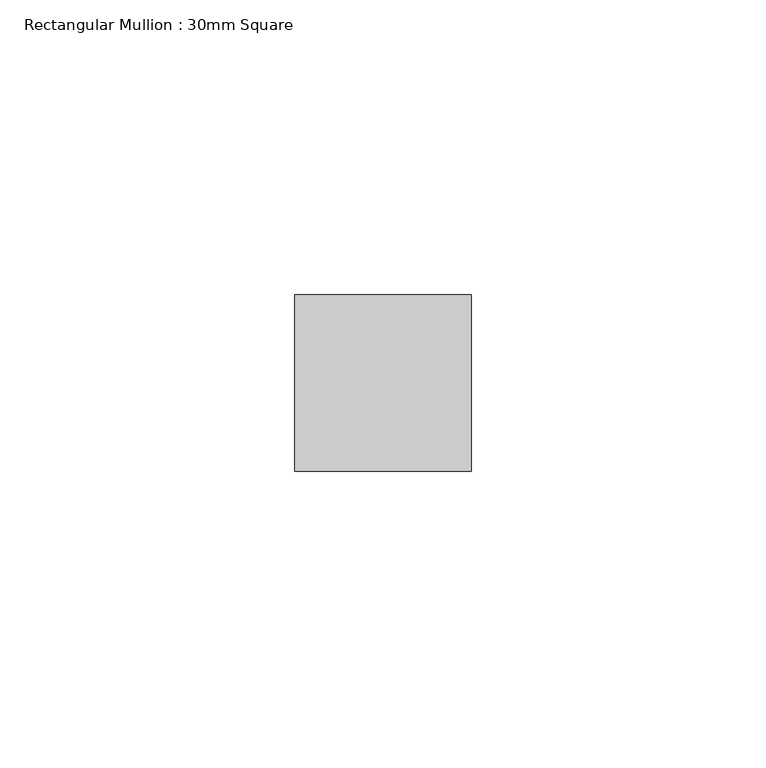
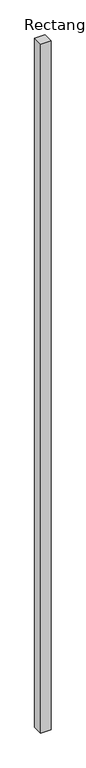
"""IFC4 building model written with IfcOpenShell, lengths in millimetres: member geometry, Rectangular Mullion : 30mm Square."""

import ifcopenshell
import ifcopenshell.guid

model = None  # the IFC model being written
_history = None  # IfcOwnerHistory: only IFC2X3 demands one
_inside = {}  # id of a spatial element -> (the spatial element, [elements in it])
_under = {}  # id of a project, library or spatial element -> (it, [spatial elements below it])
_declared = {}  # id of a project -> (the project, [libraries it declares])
_typed = {}  # id of a type object -> (the type object, [elements of that type])
_made_of = {}  # id of a material, layer set ... -> (it, [elements and type objects made of it])


def new_model(schema):
    """Start an empty IFC model of exactly this schema.

    Asked for "IFC4X3", IfcOpenShell would pick the latest addendum, in which some entities
    have other attributes; the version numbers below select the first issue.
    IFC2X3 requires an IfcOwnerHistory on every rooted entity: one is made here for all.
    """
    global model, _history
    if schema == "IFC4X3":
        model = ifcopenshell.file(schema_version=(4, 3, 0, 0))
    else:
        model = ifcopenshell.file(schema=schema)
    _inside.clear()
    _under.clear()
    _declared.clear()
    _typed.clear()
    _made_of.clear()
    _history = None
    if model.schema == "IFC2X3":
        org = make("IfcOrganization", Name="unknown")
        user = make(
            "IfcPersonAndOrganization",
            ThePerson=make("IfcPerson", FamilyName="unknown"),
            TheOrganization=org,
        )
        app = make(
            "IfcApplication",
            ApplicationDeveloper=org,
            Version="unknown",
            ApplicationFullName="unknown",
            ApplicationIdentifier="unknown",
        )
        _history = make(
            "IfcOwnerHistory",
            OwningUser=user,
            OwningApplication=app,
            ChangeAction="ADDED",
            CreationDate=0,
        )
    return model


def make(cls, **values):
    """One entity of the class cls with the attributes given. An attribute that is None is left unset."""
    return model.create_entity(
        cls, **{name: value for name, value in values.items() if value is not None}
    )


def rooted(cls, **values):
    """An entity with a GlobalId (a new one), such as an element, a storey or a relation."""
    return make(cls, GlobalId=ifcopenshell.guid.new(), OwnerHistory=_history, **values)


def si_unit(unit_type, name, prefix=None):
    """IfcSIUnit, for example si_unit("LENGTHUNIT", "METRE", prefix="MILLI")."""
    return make("IfcSIUnit", UnitType=unit_type, Prefix=prefix, Name=name)


def assignment(units):
    """IfcUnitAssignment: the units of a project."""
    return None if units is None else make("IfcUnitAssignment", Units=units)


def point(xyz):
    """IfcCartesianPoint."""
    return None if xyz is None else make("IfcCartesianPoint", Coordinates=xyz)


def direction(xyz):
    """IfcDirection."""
    return None if xyz is None else make("IfcDirection", DirectionRatios=xyz)


def frame(location, z_axis=None, x_axis=None):
    """IfcAxis2Placement3D, a coordinate frame: its origin and axes. An axis left out is left unset."""
    return make(
        "IfcAxis2Placement3D",
        Location=point(location),
        Axis=direction(z_axis),
        RefDirection=direction(x_axis),
    )


def origin():
    """The frame at (0, 0, 0) with its axes left unset."""
    return frame((0.0, 0.0, 0.0))


def place(relative_to, where):
    """IfcLocalPlacement: puts the frame where relative to a parent placement (None: the world)."""
    return make(
        "IfcLocalPlacement", PlacementRelTo=relative_to, RelativePlacement=where
    )


def context(
    kind, dimensions, precision=None, world=None, true_north=None, identifier=None
):
    """IfcGeometricRepresentationContext, for example the 3D "Model" context."""
    return make(
        "IfcGeometricRepresentationContext",
        ContextIdentifier=identifier,
        ContextType=kind,
        CoordinateSpaceDimension=dimensions,
        Precision=precision,
        WorldCoordinateSystem=world,
        TrueNorth=true_north,
    )


def project(units=None, contexts=None):
    """IfcProject with its units and contexts."""
    return rooted(
        "IfcProject",
        Name="project",
        RepresentationContexts=contexts,
        UnitsInContext=assignment(units),
    )


def spatial(cls, under=None, at=None, **own):
    """A site, building, storey or space (cls), placed at a placement, below another one or the project."""
    s = rooted(cls, ObjectPlacement=at, **own)
    if under is not None:
        _under.setdefault(under.id(), (under, []))[1].append(s)
    return s


def polyline(points):
    """IfcPolyline through the points."""
    return make("IfcPolyline", Points=[point(p) for p in points])


def outline(outer, holes=None, kind="AREA"):
    """IfcArbitraryClosedProfileDef: a profile drawn as a closed curve; with holes, ...WithVoids."""
    if holes is None:
        return make("IfcArbitraryClosedProfileDef", ProfileType=kind, OuterCurve=outer)
    return make(
        "IfcArbitraryProfileDefWithVoids",
        ProfileType=kind,
        OuterCurve=outer,
        InnerCurves=holes,
    )


def extrude(swept, where, along, depth):
    """IfcExtrudedAreaSolid: the profile swept, set in the frame where, extruded along a direction by depth."""
    return make(
        "IfcExtrudedAreaSolid",
        SweptArea=swept,
        Position=where,
        ExtrudedDirection=direction(along),
        Depth=depth,
    )


def shape(context_of_items, identifier, shape_type, items):
    """IfcShapeRepresentation: the items that make up one representation, for example the "Body"."""
    return make(
        "IfcShapeRepresentation",
        ContextOfItems=context_of_items,
        RepresentationIdentifier=identifier,
        RepresentationType=shape_type,
        Items=items,
    )


def source(mapping_origin, context_of_items, identifier, shape_type, items):
    """IfcRepresentationMap: a shape defined once, which mapped items show again and again."""
    return make(
        "IfcRepresentationMap",
        MappingOrigin=mapping_origin,
        MappedRepresentation=shape(context_of_items, identifier, shape_type, items),
    )


def transform(
    local_origin,
    x_axis=None,
    y_axis=None,
    z_axis=None,
    scale=None,
    scale2=None,
    scale3=None,
    uniform=True,
):
    """IfcCartesianTransformationOperator3D, or its non-uniform kind. x_axis, y_axis, z_axis: its Axis1, 2, 3."""
    if uniform:
        return make(
            "IfcCartesianTransformationOperator3D",
            Axis1=direction(x_axis),
            Axis2=direction(y_axis),
            LocalOrigin=point(local_origin),
            Scale=scale,
            Axis3=direction(z_axis),
        )
    return make(
        "IfcCartesianTransformationOperator3DnonUniform",
        Axis1=direction(x_axis),
        Axis2=direction(y_axis),
        LocalOrigin=point(local_origin),
        Scale=scale,
        Axis3=direction(z_axis),
        Scale2=scale2,
        Scale3=scale3,
    )


def mapped(mapping_source, mapping_target):
    """IfcMappedItem: shows the shape of a source again, moved by a transform."""
    return make(
        "IfcMappedItem", MappingSource=mapping_source, MappingTarget=mapping_target
    )


def made_of(thing, what):
    """Note that an element or type object is made of a material, layer set ...; save() writes the relation."""
    if what is not None:
        _made_of.setdefault(what.id(), (what, []))[1].append(thing)
    return thing


def element(
    cls,
    number,
    at=None,
    inside=None,
    cuts=None,
    type_object=None,
    material=None,
    context=None,
    identifier="Body",
    shape_type=None,
    held_by="IfcProductDefinitionShape",
    body=None,
    shapes=None,
    **own,
):
    """One element of the class cls, such as IfcWall. Its Tag is "e" and its number.

    at: its placement. inside: the storey or other place that contains it. cuts: it is an
    opening in that element (IfcRelVoidsElement). A single representation is given by context,
    identifier, shape_type and body (its items); several are given by shapes. held_by: the class
    of the entity that holds the representations. save() writes the other relations.
    """
    e = rooted(cls, Tag="e%d" % number, ObjectPlacement=at, **own)
    if body is not None:
        shapes = [shape(context, identifier, shape_type, body)]
    if shapes is not None:
        e.Representation = make(held_by, Representations=shapes)
    if inside is not None:
        _inside.setdefault(inside.id(), (inside, []))[1].append(e)
    if cuts is not None:
        rooted(
            "IfcRelVoidsElement", RelatingBuildingElement=cuts, RelatedOpeningElement=e
        )
    if type_object is not None:
        _typed.setdefault(type_object.id(), (type_object, []))[1].append(e)
    return made_of(e, material)


def aggregate(whole, parts):
    """IfcRelAggregates: a whole, such as a stair, and the parts it consists of."""
    return rooted("IfcRelAggregates", RelatingObject=whole, RelatedObjects=parts)


def save(model, path):
    """Write the relations noted so far, then the file.

    IfcRelAggregates (storeys below a building ...), IfcRelContainedInSpatialStructure (elements
    in a storey), IfcRelDefinesByType, IfcRelAssociatesMaterial and IfcRelDeclares: one each for
    every whole, place, type object, material and project.
    """
    for whole, parts in _under.values():
        aggregate(whole, parts)
    for where, things in _inside.values():
        rooted(
            "IfcRelContainedInSpatialStructure",
            RelatedElements=things,
            RelatingStructure=where,
        )
    for kind, things in _typed.values():
        rooted("IfcRelDefinesByType", RelatedObjects=things, RelatingType=kind)
    for what, things in _made_of.values():
        rooted("IfcRelAssociatesMaterial", RelatedObjects=things, RelatingMaterial=what)
    for by, libraries in _declared.values():
        rooted("IfcRelDeclares", RelatingContext=by, RelatedDefinitions=libraries)
    model.write(path)


def rectangular_mullion_30mm_square_a1c2493b(model_context):
    return source(origin(), model_context, "Body", "SweptSolid", [
        extrude(outline(polyline([(15.0, 15.0), (15.0, -15.0), (-15.0, -15.0), (-15.0, 15.0), (15.0, 15.0)])), frame((0.0, 0.0, -2124.2685603), z_axis=(0.0, 0.0, 1.0), x_axis=(1.0, 0.0, 0.0)), (0.0, 0.0, 1.0), 2124.2685603),
    ])


if __name__ == "__main__":
    model = new_model("IFC4")
    model_context = context("Model", 3, world=origin())
    ifc_project = project(units=[si_unit("LENGTHUNIT", "METRE", prefix="MILLI")], contexts=[model_context])
    site = spatial("IfcSite", under=ifc_project)
    building = spatial("IfcBuilding", under=site)
    placement = place(None, origin())
    rectangular_mullion_30mm_square_shape = rectangular_mullion_30mm_square_a1c2493b(model_context)
    element("IfcMember", 1, ObjectType="Rectangular Mullion : 30mm Square", at=placement, inside=building, context=model_context, shape_type="MappedRepresentation", body=[
        mapped(rectangular_mullion_30mm_square_shape, transform((0.0, 0.0, 0.0), x_axis=(1.0, 0.0, 0.0), y_axis=(0.0, 1.0, 0.0), z_axis=(0.0, 0.0, 1.0))),
    ])
    save(model, "model.ifc")

# Revit data of these elements
# Type "Rectangular Mullion : 30mm Square"
#   built-in parameter 1007304 = 0.0984252 (stored number, unit not read)
#   built-in parameter 1007301 = 0.0492126 (stored number, unit not read)
#   built-in parameter 1007300 = 0.0492126 (stored number, unit not read)
# Element 1 (IfcMember, "Rectangular Mullion : 30mm Square")
#   Materials on its faces: "Aluminum"
# Materials
#   "Aluminum": class "Metal", colour RGB 244 244 244, transparency 0, Description = "Aluminum 6061", Cost = 0
